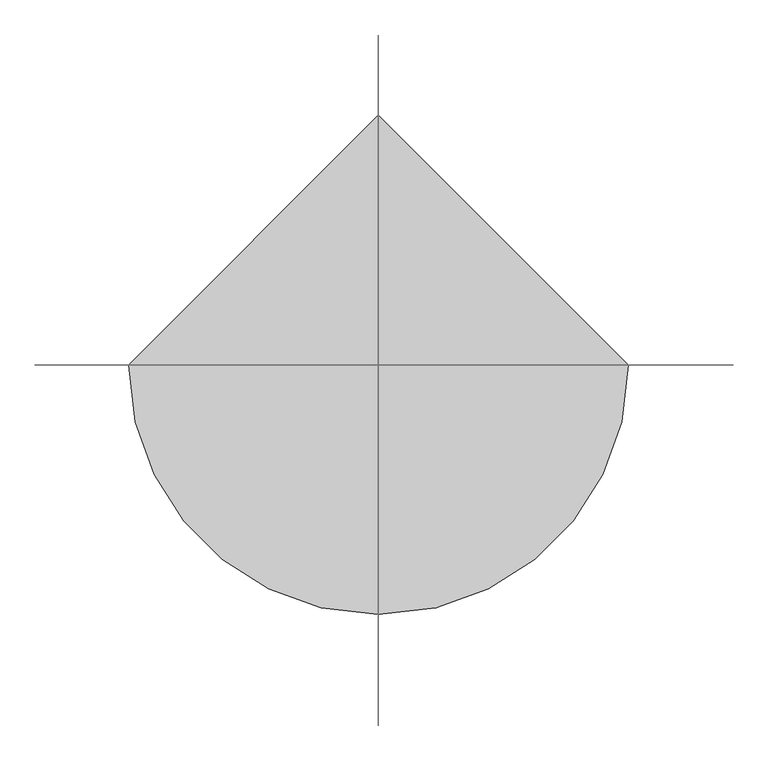
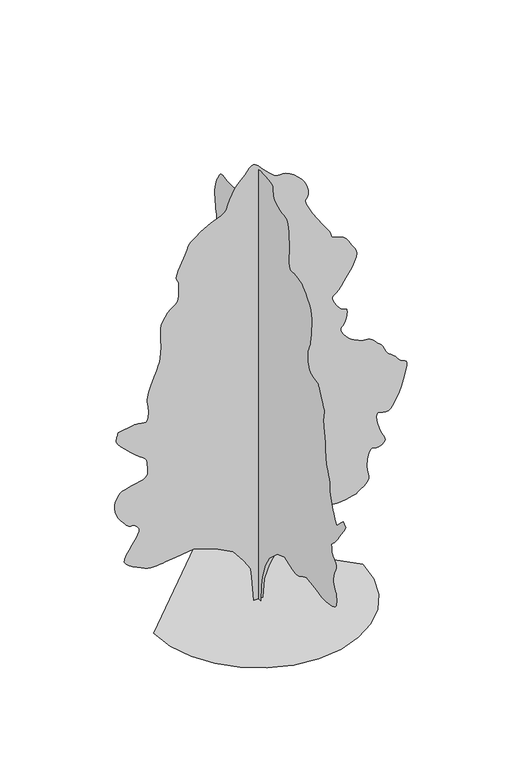
"""IFC4 building model written with IfcOpenShell, lengths in millimetres: geographic element geometry, RPC 木 - 落葉樹 : セイヨウハコヤナギ - 12.2 メートル."""

from ifc_helpers import new_model, si_unit, origin, place, context, project, spatial, triangles, source, transform, mapped, element, save


def geographic_element_e292760b(model_context):
    return source(origin(), model_context, "Body", "Tessellation", [
        triangles([(0.0009702, 113.8903775, 0.0), (0.0009702, -104.9033079, 0.0), (0.0009702, -123.1361794, 437.5878977), (0.0009702, -177.8345485, 729.312315), (0.0009702, -323.695976, 1130.4323805), (0.0009702, -506.0246724, 1440.3907139), (0.0009702, -870.6795582, 1768.5802746), (0.0009702, -1217.1031076, 1896.2099842), (0.0009702, -1399.4317314, 1823.2794067), (0.0009702, -1477.3592422, 1796.3301796), (0.0009702, -1554.013139, 1771.7701962), (0.0009702, -1628.1128311, 1751.9959671), (0.0009702, -1698.3871754, 1739.3994976), (0.0009702, -1763.5554359, 1736.3672699), (0.0009702, -1822.3466148, 1745.2987015), (0.0009702, -1873.4849178, 1768.5802746), (0.0009702, -1920.3683933, 1798.2415455), (0.0009702, -1967.2544849, 1825.0332241), (0.0009702, -2014.1379604, 1849.4331882), (0.0009702, -2061.0214359, 1871.9166996), (0.0009702, -2107.9050568, 1892.969339), (0.0009702, -2154.791003, 1913.0611359), (0.0009702, -2201.6746239, 1932.6776711), (0.0009702, -2584.5657875, 1877.9785389), (0.0009702, -2650.9541771, 1862.4566666), (0.0009702, -2717.1899597, 1847.5726913), (0.0009702, -2783.0952393, 1833.9646557), (0.0009702, -2848.5429886, 1822.2704567), (0.0009702, -2913.3300224, 1813.1255207), (0.0009702, -2977.329023, 1807.1729771), (0.0009702, -3040.387674, 1805.045636), (0.0009702, -3113.6893044, 1807.4372051), (0.0009702, -3202.6219574, 1815.2528618), (0.0009702, -3298.2393768, 1829.4456001), (0.0009702, -3391.6453033, 1850.9733559), (0.0009702, -3473.8681915, 1880.7947914), (0.0009702, -3536.0117821, 1919.8652264), (0.0009702, -3569.1298187, 1969.1428871), (0.0009702, -3581.5837097, 2022.7771133), (0.0009702, -3588.2684761, 2074.4973576), (0.0009702, -3590.1747551, 2124.6265652), (0.0009702, -3588.2684761, 2173.4773624), (0.0009702, -3583.4899887, 2221.3724041), (0.0009702, -3576.7802238, 2268.6270779), (0.0009702, -3569.1298187, 2315.5638931), (0.0009702, -3534.359848, 2355.0613369), (0.0009702, -3502.0042648, 2397.1080437), (0.0009702, -3474.4018799, 2444.2583633), (0.0009702, -3453.9923698, 2499.0617043), (0.0009702, -3443.1648331, 2564.0801193), (0.0009702, -3444.2577896, 2641.8294434), (0.0009702, -3459.736496, 2734.9307373), (0.0009702, -3486.8051926, 2827.040522), (0.0009702, -3517.6864471, 2902.5786438), (0.0009702, -3547.2968491, 2965.0274483), (0.0009702, -3570.5276985, 3017.919278), (0.0009702, -3582.270005, 3064.7620583), (0.0009702, -3577.4156502, 3109.0378441), (0.0009702, -3550.9059311, 3154.2795593), (0.0009702, -3512.094928, 3195.2003174), (0.0009702, -3474.8849899, 3227.1998177), (0.0009702, -3440.8774727, 3254.7513336), (0.0009702, -3411.622863, 3282.2775604), (0.0009702, -3388.7733856, 3314.2770607), (0.0009702, -3373.8792366, 3355.1981094), (0.0009702, -3368.5670609, 3409.5386879), (0.0009702, -3364.9071098, 3462.7866005), (0.0009702, -3357.1040977, 3500.758992), (0.0009702, -3349.9112228, 3528.1834808), (0.0009702, -3348.1575508, 3549.8638435), (0.0009702, -3356.6212784, 3570.6038567), (0.0009702, -3380.0553131, 3595.1564278), (0.0009702, -3423.2637222, 3628.3250427), (0.0009702, -3483.805957, 3682.2845398), (0.0009702, -3554.8963852, 3763.0330994), (0.0009702, -3634.7298843, 3866.097448), (0.0009702, -3721.578653, 3987.029892), (0.0009702, -3813.7140175, 4121.3568672), (0.0009702, -3909.3311462, 4264.6048096), (0.0009702, -4006.7278175, 4412.3263161), (0.0009702, -3897.3344948, 4521.744928), (0.0009702, -3751.468689, 4394.1024284), (0.0009702, -3605.6025925, 4230.012735), (0.0009702, -3582.0921089, 4261.5802849), (0.0009702, -3558.302282, 4295.0794029), (0.0009702, -3533.825869, 4332.3910789), (0.0009702, -3508.4346863, 4375.4468811), (0.0009702, -3481.7473618, 4426.1527977), (0.0009702, -3453.4586815, 4486.4412689), (0.0009702, -3423.2637222, 4558.1924126), (0.0009702, -3392.2298607, 4631.6207794), (0.0009702, -3362.4671425, 4698.9495186), (0.0009702, -3335.2458389, 4765.3631973), (0.0009702, -3311.8626732, 4835.8943573), (0.0009702, -3293.5626274, 4915.6772781), (0.0009702, -3281.6677139, 5009.820369), (0.0009702, -3277.3976257, 5123.4070404), (0.0009702, -3269.2135323, 5238.2901443), (0.0009702, -3247.6349075, 5336.8812195), (0.0009702, -3217.1347343, 5425.3060547), (0.0009702, -3182.1615784, 5509.5363785), (0.0009702, -3147.1628426, 5595.7241409), (0.0009702, -3116.6629601, 5689.8422333), (0.0009702, -3095.0843353, 5798.0408615), (0.0009702, -3081.5880661, 5895.9965103), (0.0009702, -3071.9043549, 5963.3505386), (0.0009702, -3065.4230644, 6011.8708328), (0.0009702, -3061.4834793, 6053.4014374), (0.0009702, -3059.4754623, 6099.6852402), (0.0009702, -3058.7130089, 6162.5657043), (0.0009702, -3058.6112709, 6253.8368774), (0.0009702, -3054.5702385, 6347.2939636), (0.0009702, -3044.1493629, 6416.5036926), (0.0009702, -3029.9159294, 6472.9537354), (0.0009702, -3014.3863541, 6528.1335068), (0.0009702, -3000.1532112, 6593.5300964), (0.0009702, -2989.7323357, 6680.582341), (0.0009702, -2985.6910126, 6800.8284897), (0.0009702, -2991.2572426, 6913.2716263), (0.0009702, -3003.5335281, 6981.3628189), (0.0009702, -3015.8351028, 7023.299794), (0.0009702, -3021.4013329, 7057.2564423), (0.0009702, -3013.5986115, 7101.4304901), (0.0009702, -2985.6910126, 7173.9952469), (0.0009702, -2930.9943512, 7293.1228592), (0.0009702, -2868.6219955, 7422.976561), (0.0009702, -2820.6353897, 7519.3561432), (0.0009702, -2784.5945663, 7587.8287079), (0.0009702, -2758.1107178, 7633.959613), (0.0009702, -2738.8194534, 7663.3671204), (0.0009702, -2724.3063858, 7681.5904266), (0.0009702, -2712.1827072, 7694.2483749), (0.0009702, -2638.2965195, 7706.295314), (0.0009702, -2566.4945068, 7720.4525894), (0.0009702, -2498.8204399, 7738.7270554), (0.0009702, -2437.3730278, 7763.2290482), (0.0009702, -2384.2142086, 7796.0415802), (0.0009702, -2341.425396, 7839.199411), (0.0009702, -2311.0702721, 7894.8105515), (0.0009702, -2290.8183105, 7956.2428482), (0.0009702, -2276.3080044, 8015.7938644), (0.0009702, -2266.578511, 8073.7182358), (0.0009702, -2260.6793072, 8130.3973343), (0.0009702, -2257.6495502, 8186.1107941), (0.0009702, -2256.5313046, 8241.1632477), (0.0009702, -2256.3736107, 8295.9104874), (0.0009702, -2287.4709858, 8351.2169952), (0.0009702, -2317.6099892, 8410.0058487), (0.0009702, -2345.8351559, 8475.8093903), (0.0009702, -2371.1907303, 8552.1355453), (0.0009702, -2392.7211021, 8642.5172379), (0.0009702, -2409.4655743, 8750.4106522), (0.0009702, -2420.4685364, 8879.374292), (0.0009702, -2431.6848576, 9010.8290588), (0.0009702, -2445.4530579, 9127.2882294), (0.0009702, -2455.3934395, 9233.8857925), (0.0009702, -2455.1265953, 9335.6789978), (0.0009702, -2438.2754436, 9437.7779984), (0.0009702, -2398.4602867, 9545.3156204), (0.0009702, -2329.3041882, 9663.375856), (0.0009702, -2249.3561611, 9774.6498779), (0.0009702, -2178.6572788, 9861.3457489), (0.0009702, -2113.0620094, 9927.9370331), (0.0009702, -2048.4224957, 9978.9234558), (0.0009702, -1980.5956764, 10018.7256775), (0.0009702, -1905.4310783, 10051.8434235), (0.0009702, -1818.7857857, 10082.7252594), (0.0009702, -1726.6658272, 10101.4566742), (0.0009702, -1639.9671947, 10102.9310028), (0.0009702, -1561.8796646, 10098.9917084), (0.0009702, -1495.593013, 10101.4566742), (0.0009702, -1444.2971615, 10122.0693695), (0.0009702, -1411.1794155, 10172.6744202), (0.0009702, -1399.4317314, 10265.0641296), (0.0009702, -1401.3457134, 10369.4751984), (0.0009702, -1405.8114292, 10455.052533), (0.0009702, -1410.9150421, 10532.0141144), (0.0009702, -1414.7402447, 10610.5767609), (0.0009702, -1415.3781418, 10700.9584534), (0.0009702, -1410.9150421, 10813.3260132), (0.0009702, -1399.4317314, 10957.9206757), (0.0009702, -1383.5921459, 11104.7268311), (0.0009702, -1366.4740047, 11219.3303009), (0.0009702, -1346.8067459, 11305.2390106), (0.0009702, -1323.3115231, 11365.9341431), (0.0009702, -1294.7128326, 11404.9480408), (0.0009702, -1259.7344444, 11425.7897919), (0.0009702, -1217.1031076, 11431.9661591), (0.0009702, -1156.2404709, 11437.4821014), (0.0009702, -1074.0049381, 11453.8752869), (0.0009702, -980.2913269, 11480.7666687), (0.0009702, -884.9789761, 11517.8748688), (0.0009702, -797.9626305, 11564.8440948), (0.0009702, -729.1241724, 11621.4220367), (0.0009702, -688.3534052, 11687.2249969), (0.0009702, -673.3092653, 11757.0707336), (0.0009702, -668.4724966, 11824.0433899), (0.0009702, -663.953441, 11885.2722107), (0.0009702, -649.8675276, 11937.9096954), (0.0009702, -616.3252436, 11979.0595093), (0.0009702, -553.4419453, 12005.8485718), (0.0009702, -451.3255766, 12015.4049652), (0.0009702, -328.0015635, 12019.0907867), (0.0009702, -210.419678, 12026.8937988), (0.0009702, -102.0858745, 12034.0608032), (0.0009702, -6.5099094, 12035.8141846), (0.0009702, 72.8000803, 12027.3763275), (0.0009702, 132.3357269, 12003.9417114), (0.0009702, 168.5887284, 11960.7083038), (0.0009702, 190.3829832, 11911.6031616), (0.0009702, 211.2205557, 11869.1836578), (0.0009702, 234.6091899, 11826.7629913), (0.0009702, 264.0584098, 11777.6322693), (0.0009702, 303.0754686, 11715.1325958), (0.0009702, 355.1693819, 11632.5283356), (0.0009702, 423.847639, 11523.1361755), (0.0009702, 499.9145439, 11406.6002655), (0.0009702, 572.4739231, 11305.3913269), (0.0009702, 642.4814959, 11216.9420746), (0.0009702, 710.8954159, 11138.6840607), (0.0009702, 778.6688227, 11068.1023224), (0.0009702, 846.7624861, 11002.602832), (0.0009702, 916.132089, 10939.6717896), (0.0009702, 984.3859171, 10887.6947296), (0.0009702, 1049.1322557, 10854.1956116), (0.0009702, 1111.3241718, 10835.3874573), (0.0009702, 1171.9250513, 10827.4065491), (0.0009702, 1231.8854176, 10826.440329), (0.0009702, 1292.1634243, 10828.6774017), (0.0009702, 1353.7199867, 10830.2784668), (0.0009702, 1420.0599781, 10835.869986), (0.0009702, 1491.5035824, 10848.1459808), (0.0009702, 1564.2205101, 10860.4231384), (0.0009702, 1634.3881748, 10865.9890778), (0.0009702, 1698.1762871, 10858.1860657), (0.0009702, 1751.7570282, 10830.2784668), (0.0009702, 1791.3078117, 10775.5818054), (0.0009702, 1825.3814587, 10707.9731415), (0.0009702, 1862.9624496, 10643.2119781), (0.0009702, 1900.8637699, 10577.5101746), (0.0009702, 1935.8928818, 10507.0295929), (0.0009702, 1964.8627705, 10427.9332581), (0.0009702, 1984.5861305, 10336.4086121), (0.0009702, 1991.8679535, 10228.5907745), (0.0009702, 1989.7406124, 10117.6475464), (0.0009702, 1983.7879234, 10017.5559814), (0.0009702, 1974.6456036, 9925.75112), (0.0009702, 1962.9514046, 9839.6912567), (0.0009702, 1949.3433689, 9756.8323608), (0.0009702, 1934.4593937, 9674.610054), (0.0009702, 1918.9375214, 9590.455307), (0.0009702, 1915.5875805, 9511.6130264), (0.0009702, 1932.3320526, 9444.2589981), (0.0009702, 1962.471056, 9384.2504517), (0.0009702, 1999.3099411, 9327.4190369), (0.0009702, 2036.1488262, 9269.6469818), (0.0009702, 2066.2878296, 9206.7659363), (0.0009702, 2083.0323017, 9134.6337112), (0.0009702, 2082.5544239, 9064.6106598), (0.0009702, 2068.0415016, 9007.7030869), (0.0009702, 2043.3239697, 8959.0554749), (0.0009702, 2012.2265945, 8913.9157883), (0.0009702, 1978.5801018, 8867.505249), (0.0009702, 1946.2069324, 8815.045079), (0.0009702, 1918.9375214, 8751.7320831), (0.0009702, 1903.0953197, 8679.3963821), (0.0009702, 1901.6083466, 8603.858551), (0.0009702, 1913.195866, 8526.4138596), (0.0009702, 1936.584264, 8448.3337418), (0.0009702, 1970.4976009, 8370.8640518), (0.0009702, 2013.6626987, 8295.3256393), (0.0009702, 2064.7983856, 8222.9899384), (0.0009702, 2117.5836811, 8163.4133423), (0.0009702, 2167.8170975, 8119.112558), (0.0009702, 2217.4124714, 8080.9114014), (0.0009702, 2268.2839302, 8039.4819534), (0.0009702, 2322.3450199, 7985.6497742), (0.0009702, 2381.5073971, 7910.1113617), (0.0009702, 2447.6872238, 7803.6411163), (0.0009702, 2517.1100212, 7689.1899628), (0.0009702, 2585.5825859, 7593.5731247), (0.0009702, 2654.3597832, 7513.2309357), (0.0009702, 2724.7386269, 7444.7333725), (0.0009702, 2797.9893883, 7384.4957703), (0.0009702, 2875.3829201, 7329.0619446), (0.0009702, 2958.2156548, 7274.8739731), (0.0009702, 3041.988739, 7232.046936), (0.0009702, 3121.6190529, 7206.7316208), (0.0009702, 3197.4115196, 7189.7280075), (0.0009702, 3269.6963516, 7171.7587555), (0.0009702, 3338.8043427, 7143.5971024), (0.0009702, 3405.0398346, 7095.9662888), (0.0009702, 3468.7339119, 7019.6145538), (0.0009702, 3527.5736343, 6926.1324692), (0.0009702, 3577.7967316, 6834.2258698), (0.0009702, 3617.5230858, 6745.496402), (0.0009702, 3644.7696785, 6661.5707108), (0.0009702, 3657.7066795, 6583.9992828), (0.0009702, 3654.3516518, 6514.4337616), (0.0009702, 3632.823896, 6454.3996353), (0.0009702, 3592.3603775, 6396.7293182), (0.0009702, 3536.9268425, 6334.585437), (0.0009702, 3471.6061203, 6270.2306442), (0.0009702, 3401.4816216, 6205.8502716), (0.0009702, 3331.6876259, 6143.7069717), (0.0009702, 3267.3072533, 6086.0366547), (0.0009702, 3213.4747833, 6035.0508133), (0.0009702, 3163.8615326, 5989.0210648), (0.0009702, 3111.4016533, 5943.6273239), (0.0009702, 3059.8821236, 5897.267363), (0.0009702, 3013.1663704, 5848.3656967), (0.0009702, 2975.0669518, 5795.3212601), (0.0009702, 2949.3705551, 5736.5324066), (0.0009702, 2939.966478, 5670.3986526), (0.0009702, 2936.1033417, 5601.0871857), (0.0009702, 2926.8007118, 5533.3517853), (0.0009702, 2915.5665138, 5466.6081848), (0.0009702, 2905.9589607, 5400.1436371), (0.0009702, 2901.4348183, 5333.3738754), (0.0009702, 2905.5270103, 5265.6640549), (0.0009702, 2921.742881, 5196.3531693), (0.0009702, 2946.7782715, 5129.7357239), (0.0009702, 2974.6855797, 5069.8289154), (0.0009702, 3004.9822769, 5015.5136261), (0.0009702, 3037.1852531, 4965.6463211), (0.0009702, 3070.8366875, 4919.1340439), (0.0009702, 3105.4543419, 4874.8579674), (0.0009702, 3140.5292358, 4831.7007179), (0.0009702, 3183.2289551, 4838.4869316), (0.0009702, 3224.1497131, 4839.2493851), (0.0009702, 3261.5631271, 4827.8625801), (0.0009702, 3293.7405235, 4798.3030472), (0.0009702, 3318.877652, 4744.5214462), (0.0009702, 3335.2458389, 4660.4178589), (0.0009702, 3341.091703, 4539.9685249), (0.0009702, 3341.091703, 3938.2808327), (0.0009702, 3347.8017586, 3760.1103127), (0.0009702, 3363.4330719, 3613.5070518), (0.0009702, 3381.2752968, 3494.3285706), (0.0009702, 3394.6701187, 3398.431517), (0.0009702, 3396.9066101, 3321.6734116), (0.0009702, 3381.2752968, 3259.8856133), (0.0009702, 3341.091703, 3208.9762207), (0.0009702, 3283.7263092, 3180.3314575), (0.0009702, 3223.8195007, 3176.2395561), (0.0009702, 3165.5137573, 3178.8321304), (0.0009702, 3112.95214, 3170.2666649), (0.0009702, 3070.2521301, 3132.7009346), (0.0009702, 3041.6076576, 3048.2159752), (0.0009702, 3031.1359131, 2899.0204308), (0.0009702, 3038.0494446, 2734.6002342), (0.0009702, 3055.1547958, 2610.6941345), (0.0009702, 3077.0639236, 2518.6782394), (0.0009702, 3098.3376251, 2449.9466789), (0.0009702, 3113.5366974, 2395.8855892), (0.0009702, 3117.2475174, 2347.8837227), (0.0009702, 3104.0561714, 2297.3325932), (0.0009702, 3091.0938812, 2255.6569393), (0.0009702, 3091.8307549, 2234.0756985), (0.0009702, 3095.4654167, 2223.657439), (0.0009702, 3091.0938812, 2215.4707294), (0.0009702, 3067.9139008, 2200.5867542), (0.0009702, 3015.0726494, 2170.0740818), (0.0009702, 2921.742881, 2115.0038967), (0.0009702, 2824.1938934, 2054.1920563), (0.0009702, 2755.3655365, 2010.2848526), (0.0009702, 2699.2709953, 1980.0923641), (0.0009702, 2639.9996132, 1960.4249599), (0.0009702, 2561.6145721, 1948.0928638), (0.0009702, 2448.1142326, 1939.9061543), (0.0009702, 2283.5922981, 1932.6776711), (0.0009702, 2107.2721012, 1934.962706), (0.0009702, 1964.7585617, 1953.194006), (0.0009702, 1849.6721272, 1980.9972507), (0.0009702, 1755.6381866, 2011.9851849), (0.0009702, 1676.2747169, 2039.7859589), (0.0009702, 1605.2047817, 2058.0197296), (0.0009702, 1536.0486832, 2060.3047646), (0.0009702, 1461.4686424, 2050.3642376), (0.0009702, 1379.2357258, 2036.5986534), (0.0009702, 1290.6232567, 2019.6406769), (0.0009702, 1196.9070293, 2000.1334373), (0.0009702, 1099.3656721, 1978.709745), (0.0009702, 999.2698923, 1956.0127293), (0.0009702, 897.9007891, 1932.6776711), (0.0009702, 533.2433599, 1640.9507103), (0.0009702, 314.4519545, 1166.90014), (0.0009702, 168.5887284, 601.6827144), (120.2564769, 0.0005338, 0.0085401), (-116.7693169, 0.0005338, 0.0085401), (-171.467677, 0.0004852, 656.3894405), (-207.9336742, 0.0004852, 911.6486418), (-390.2621163, 0.000461, 1203.3730591), (-663.7526539, 0.0004367, 1549.7965359), (-1137.8057676, 0.0004124, 1805.0556644), (-1721.2571457, 0.0004124, 1987.3818901), (-2195.307716, 0.0004124, 1932.6853741), (-2468.8007607, 0.0004124, 1896.220158), (-2535.4583199, 0.0004124, 1886.7041691), (-2609.1436478, 0.0004124, 1875.9122406), (-2687.9097702, 0.0004124, 1867.0367649), (-2769.8786041, 0.0004124, 1863.262286), (-2853.118, 0.0004124, 1867.7814869), (-2935.7219696, 0.0004124, 1883.781237), (-3015.7842339, 0.0004124, 1914.451458), (-3106.3182426, 0.0004124, 1956.8718338), (-3213.0937019, 0.0004124, 2005.9868591), (-3323.4017944, 0.0004124, 2061.8043823), (-3424.4581261, 0.0004124, 2124.316555), (-3503.5038826, 0.0003882, 2193.5259933), (-3547.7796684, 0.0003882, 2269.4326973), (-3544.5263786, 0.0003882, 2352.039283), (-3497.4801224, 0.0003882, 2448.838607), (-3427.1777275, 0.0003882, 2561.589283), (-3345.9972176, 0.0003639, 2681.6572449), (-3266.4177727, 0.0003639, 2800.4802246), (-3200.8682854, 0.0003639, 2909.3904373), (-3161.8029373, 0.0003397, 2999.797419), (-3161.6503304, 0.0003397, 3063.1101242), (-3185.0843651, 0.0003397, 3105.2255768), (-3208.5186905, 0.0003397, 3138.699115), (-3231.9783051, 0.0003397, 3165.0306473), (-3255.4123398, 0.0003397, 3185.5927643), (-3278.8463745, 0.0003397, 3201.8595039), (-3302.3059891, 0.0003397, 3215.2540352), (-3325.7400238, 0.0003397, 3227.2253975), (-3349.3522453, 0.0003397, 3223.6924736), (-3373.9045258, 0.0003397, 3222.5995171), (-3400.3633759, 0.0003397, 3226.2594681), (-3429.7194328, 0.0003397, 3237.112294), (-3462.8883385, 0.0003397, 3257.521804), (-3500.8351501, 0.0003397, 3289.8770966), (-3544.5263786, 0.0003397, 3336.6184296), (-3595.9950394, 0.0003397, 3397.7455124), (-3652.5471107, 0.0003154, 3470.6657707), (-3708.1585419, 0.0003154, 3553.8034286), (-3756.729705, 0.0003154, 3645.5574211), (-3792.2368401, 0.0003154, 3744.3263924), (-3808.6306068, 0.0002911, 3848.5092773), (-3799.7855072, 0.0002911, 3956.5300095), (-3773.9115051, 0.0002911, 4054.2313133), (-3742.2677971, 0.0002911, 4130.8879715), (-3703.6343994, 0.0002911, 4189.9817482), (-3656.6898811, 0.0002669, 4235.0708565), (-3600.1886787, 0.0002669, 4269.6120621), (-3532.8346504, 0.0002669, 4297.163578), (-3453.3825233, 0.0002669, 4321.1821701), (-3359.0103767, 0.0002669, 4341.1597298), (-3254.4719902, 0.0002669, 4358.2906609), (-3149.5775208, 0.0002669, 4378.5984329), (-3054.2650246, 0.0002669, 4408.1579659), (-2978.4219795, 0.0002669, 4453.018309), (-2931.9094116, 0.0002669, 4519.2540916), (-2924.6147987, 0.0002669, 4612.9143631), (-2935.5184937, 0.0002426, 4710.7174049), (-2940.34785, 0.0002426, 4788.1112274), (-2944.2365662, 0.0002426, 4849.2380196), (-2952.2680527, 0.0002426, 4898.2411331), (-2969.5260109, 0.0002426, 4939.289209), (-3001.1697189, 0.0002426, 4976.499147), (-3052.2572983, 0.0002426, 5014.0392975), (-3137.5552895, 0.0002184, 5075.3698563), (-3257.0134048, 0.0002184, 5172.1052307), (-3393.3483971, 0.0002184, 5290.5468384), (-3529.3781754, 0.0002184, 5416.9437744), (-3647.8703613, 0.0001941, 5537.6218735), (-3731.5928673, 0.0001941, 5638.8308121), (-3763.3380226, 0.0001941, 5706.8714264), (-3761.7369576, 0.0001941, 5751.0960526), (-3757.2636841, 0.0001941, 5790.5430634), (-3750.4010216, 0.0001941, 5825.9990387), (-3741.6323708, 0.0001698, 5858.2528839), (-3731.4402603, 0.0001698, 5888.1429199), (-3720.2825111, 0.0001698, 5916.4057297), (-3708.6416519, 0.0001698, 5943.906958), (-3271.0436531, 0.0001698, 6016.8269257), (-3176.2139763, 0.0001698, 6018.4285721), (-3095.0843353, 0.0001698, 6002.7969681), (-3028.0096504, 0.0001698, 5986.1997253), (-2975.270137, 0.0001698, 5984.929454), (-2937.2215874, 0.0001698, 6015.2258606), (-2914.1433449, 0.0001698, 6093.3821365), (-2906.3912018, 0.0001698, 6235.6135712), (-2912.8724922, 0.0001456, 6381.32677), (-2927.0041878, 0.0001456, 6474.7326965), (-2940.8306694, 0.0001456, 6539.4182831), (-2946.3716103, 0.0001456, 6598.9948792), (-2935.6202316, 0.0001213, 6677.0999954), (-2900.6470757, 0.0001213, 6797.269986), (-2833.4453636, 0.0001213, 6983.1673599), (-2756.1535698, 9.7e-05, 7180.2733521), (-2695.1535141, 9.7e-05, 7329.8496872), (-2648.7935532, 9.7e-05, 7449.1301971), (-2615.5232002, 7.28e-05, 7555.3463882), (-2593.7158104, 7.28e-05, 7665.7053497), (-2581.8208969, 7.28e-05, 7797.4141708), (-2578.186235, 4.85e-05, 7967.7311005), (-2581.6938698, 4.85e-05, 8141.3013199), (-2588.4036346, 4.85e-05, 8277.8644958), (-2592.5466957, 2.43e-05, 8387.3083969), (-2588.4036346, 2.43e-05, 8479.5457901), (-2570.2309067, 2.43e-05, 8564.4371201), (-2532.2710144, 2.43e-05, 8651.8701553), (-2468.8007607, 0.0, 8751.757663), (-2395.1256065, 0.0, 8844.6043213), (-2330.3792679, 0.0, 8909.7218582), (-2274.5643608, 0.0, 8955.0650208), (-2227.6808853, 0.0, 8988.6152985), (-2189.7262253, 0.0, 9018.3274384), (-2160.7029968, 0.0, 9052.1823486), (-2140.6085838, 0.0, 9098.1609375), (-2127.1072277, -2.43e-05, 9141.3437668), (-2117.4336903, -2.43e-05, 9168.8699936), (-2110.9473129, -2.43e-05, 9191.9482361), (-2107.0154308, -2.43e-05, 9221.7109543), (-2104.9947693, -2.43e-05, 9269.3417679), (-2104.2500473, -2.43e-05, 9345.9981354), (-2104.1458385, -2.43e-05, 9462.838678), (-2114.4574184, -4.85e-05, 9573.8330658), (-2137.5281033, -4.85e-05, 9640.805722), (-2161.5543983, -4.85e-05, 9686.7337326), (-2174.7354252, -4.85e-05, 9734.5680222), (-2165.2753922, -4.85e-05, 9807.2850952), (-2121.3657177, -7.28e-05, 9927.8358765), (-2031.2129356, -7.28e-05, 10119.1974518), (-1940.7398243, -7.28e-05, 10312.5926239), (-1890.135355, -9.7e-05, 10438.3535522), (-1858.9847855, -9.7e-05, 10518.2126312), (-1826.8784603, -9.7e-05, 10573.7987732), (-1773.4019279, -9.7e-05, 10626.8687897), (-1678.1453876, -9.7e-05, 10699.0527557), (-1520.6945332, -0.0001213, 10812.0551605), (-1342.5671791, -0.0001213, 10924.4727173), (-1196.3326458, -0.0001213, 10992.5894897), (-1078.165658, -0.0001213, 11034.5264648), (-984.2359989, -0.0001213, 11068.4836945), (-910.7209368, -0.0001213, 11112.6577423), (-853.7901821, -0.0001456, 11185.2219177), (-809.6161343, -0.0001456, 11304.34953), (-760.4450804, -0.0001456, 11447.9791351), (-695.3276888, -0.0001698, 11580.450119), (-620.643512, -0.0001698, 11699.5021545), (-542.7695226, -0.0001698, 11802.9470032), (-468.082766, -0.0001698, 11888.5255005), (-402.9678815, -0.0001698, 11954.0238281), (-353.7969003, -0.0001941, 11997.1816589), (-315.471151, -0.0001941, 12037.7466248), (-277.1428946, -0.0001941, 12089.4690491), (-236.5850686, -0.0001941, 12141.1914734), (-191.5607819, -0.0001941, 12181.7564392), (-139.8392296, -0.0001941, 12199.9809082), (-79.1872813, -0.0001941, 12184.7306763), (-7.3724481, -0.0001941, 12124.8238678), (68.5354242, -0.0001941, 12043.2102448), (139.978002, -0.0001941, 11969.908905), (206.9556453, -0.0001698, 11904.2582611), (269.4670731, -0.0001698, 11845.6467224), (327.5160916, -0.0001698, 11793.3906097), (381.0969054, -0.0001698, 11746.8783325), (430.2145105, -0.0001698, 11705.4750458), (477.6292399, -0.0001698, 11680.1091522), (528.236289, -0.0001698, 11674.5176331), (585.2203471, -0.0001698, 11677.2372345), (651.7712631, -0.0001698, 11676.7535431), (731.0813204, -0.0001698, 11661.6056305), (826.3377153, -0.0001698, 11620.3035004), (940.7328403, -0.0001456, 11541.3594818), (1053.7962152, -0.0001456, 11441.8539276), (1144.2183849, -0.0001456, 11345.8551361), (1213.9057011, -0.0001456, 11252.3980499), (1264.7770145, -0.0001456, 11160.5420288), (1298.7438366, -0.0001213, 11069.3220154), (1317.7198586, -0.0001213, 10977.7962067), (1323.6216785, -0.0001213, 10884.9751282), (1311.5004707, -0.0001213, 10814.3933899), (1284.7112629, -0.0001213, 10775.7085419), (1257.5994003, -0.0001213, 10747.1916779), (1244.5225822, -9.7e-05, 10707.2371399), (1259.8335663, -9.7e-05, 10634.0881165), (1317.8800232, -9.7e-05, 10506.0889526), (1433.0173267, -7.28e-05, 10301.536322), (1569.3648182, -7.28e-05, 10081.0474548), (1682.1104073, -4.85e-05, 9912.86586), (1772.2123203, -4.85e-05, 9786.7735565), (1840.6236969, -4.85e-05, 9692.579306), (1888.3053795, -4.85e-05, 9620.0657089), (1916.212833, -4.85e-05, 9559.0403641), (1925.3042839, -2.43e-05, 9499.2858719), (1944.8650085, -2.43e-05, 9450.4859436), (1996.9589218, -2.43e-05, 9421.4603897), (2071.6965111, -2.43e-05, 9400.7459564), (2159.1932053, -2.43e-05, 9376.8288116), (2249.5594917, -2.43e-05, 9338.2207031), (2332.9107994, -2.43e-05, 9273.4845383), (2399.3574703, -2.43e-05, 9171.106485), (2456.2346672, 0.0, 9061.1794739), (2512.7942963, 0.0, 8974.8393951), (2562.0212334, 0.0, 8902.2240601), (2596.892942, 0.0, 8833.4468628), (2610.3892113, 0.0, 8758.594455), (2595.4950623, 2.43e-05, 8667.8063919), (2545.2208054, 2.43e-05, 8551.1949051), (2482.9731514, 2.43e-05, 8437.658812), (2433.4843117, 2.43e-05, 8355.0295532), (2391.6486385, 2.43e-05, 8291.8944534), (2352.3646992, 4.85e-05, 8236.7152634), (2310.5314968, 4.85e-05, 8178.0281479), (2261.0426571, 4.85e-05, 8104.3454361), (2198.7948578, 4.85e-05, 8004.2038742), (2128.4161594, 4.85e-05, 7909.2218811), (2062.1829929, 7.28e-05, 7849.3150726), (2006.4749107, 7.28e-05, 7810.4529099), (1967.6687038, 7.28e-05, 7778.6060165), (1952.1468315, 7.28e-05, 7739.7438538), (1966.2887009, 7.28e-05, 7679.8370453), (2016.4686321, 7.28e-05, 7584.8550522), (2082.0105618, 7.28e-05, 7483.0612656), (2138.9412437, 9.7e-05, 7408.9971817), (2188.6943115, 9.7e-05, 7358.0880798), (2232.7108109, 9.7e-05, 7325.6563385), (2272.4166721, 9.7e-05, 7307.1022385), (2309.2555573, 9.7e-05, 7297.7993179), (2344.6583382, 9.7e-05, 7293.1228592), (2348.379332, 9.7e-05, 7265.4187363), (2350.9845509, 9.7e-05, 7235.6560181), (2351.3556038, 9.7e-05, 7201.7499481), (2348.379332, 9.7e-05, 7161.617514), (2340.9373444, 9.7e-05, 7113.1983765), (2327.913866, 0.0001213, 7054.4101044), (2308.1931221, 0.0001213, 6983.1673599), (2279.3274422, 0.0001213, 6918.9648834), (2244.722723, 0.0001213, 6875.7820541), (2212.0318405, 0.0001213, 6843.4776306), (2188.9078159, 0.0001213, 6811.7830536), (2183.0086121, 0.0001213, 6770.5315018), (2201.984634, 0.0001213, 6709.5061569), (2253.4939899, 0.0001456, 6618.5146179), (2323.6616547, 0.0001456, 6523.7872604), (2392.871093, 0.0001456, 6454.5775314), (2460.1666946, 0.0001456, 6405.1421768), (2524.592704, 0.0001456, 6369.7367798), (2585.2012138, 0.0001456, 6342.6175049), (2641.0161209, 0.0001456, 6318.0649338), (2691.0869019, 0.0001456, 6290.3096512), (2740.0394371, 0.0001456, 6267.8924149), (2792.4993164, 0.0001456, 6258.2087036), (2847.5261902, 0.0001698, 6253.9641953), (2904.1291306, 0.0001698, 6247.7878281), (2961.3927864, 0.0001698, 6232.3852798), (3018.3259392, 0.0001698, 6200.3860703), (3073.9629501, 0.0001698, 6144.4691345), (3123.5000427, 0.0001698, 6088.0696701), (3164.4460899, 0.0001698, 6052.7154327), (3199.3177986, 0.0001698, 6028.2134399), (3230.6818726, 0.0001698, 6004.3474548), (3261.0803078, 0.0001698, 5970.8989151), (3293.079808, 0.0001698, 5917.7021622), (3329.2220787, 0.0001941, 5834.5136353), (3369.5329903, 0.0001941, 5750.0798355), (3412.6902397, 0.0001941, 5692.7903091), (3459.3554146, 0.0001941, 5651.7428146), (3510.1630692, 0.0001941, 5616.1339417), (3565.774791, 0.0001941, 5575.0858658), (3626.8001358, 0.0001941, 5517.7969208), (3693.87453, 0.0002184, 5433.3881195), (3762.397673, 0.0002184, 5358.4345551), (3824.5412636, 0.0002184, 5322.6989456), (3876.1625313, 0.0002184, 5305.161644), (3913.0928352, 0.0002184, 5284.7518433), (3931.240274, 0.0002184, 5240.4254791), (3926.3859192, 0.0002184, 5151.1111633), (3894.4369972, 0.0002426, 4995.7904114), (3842.409359, 0.0002426, 4804.5811523), (3781.7398064, 0.0002669, 4624.8601456), (3715.0464935, 0.0002669, 4461.4058784), (3644.8205475, 0.0002669, 4318.9965477), (3573.6539612, 0.0002911, 4202.4356392), (3504.0631508, 0.0002911, 4116.4766418), (3438.6154015, 0.0002911, 4065.9230415), (3370.8038429, 0.0002911, 4054.7144234), (3297.8580048, 0.0002911, 4069.9643646), (3228.1148781, 0.0002911, 4091.2889351), (3169.8600037, 0.0002911, 4098.2530449), (3131.379213, 0.0002911, 4070.447184), (3120.9583374, 0.0002911, 3987.4618423), (3146.9087883, 0.0002911, 3828.8875099), (3198.9364265, 0.0003154, 3650.9204659), (3255.1327057, 0.0003154, 3516.9748627), (3306.2199944, 0.0003154, 3417.4687271), (3342.947113, 0.0003397, 3342.8200859), (3356.0620102, 0.0003397, 3283.4975441), (3336.3643753, 0.0003397, 3229.9194191), (3274.525708, 0.0003397, 3172.5031563), (3194.0056229, 0.0003397, 3136.3100166), (3123.6779388, 0.0003397, 3137.4282623), (3062.601725, 0.0003397, 3152.9069687), (3009.8113426, 0.0003397, 3159.7696312), (2964.3664421, 0.0003397, 3135.039164), (2925.3010941, 0.0003397, 3055.7902222), (2891.6496597, 0.0003639, 2899.0204308), (2877.9754944, 0.0003639, 2720.9007797), (2889.5146156, 0.0003882, 2585.811351), (2911.2458473, 0.0003882, 2483.2830162), (2928.2241714, 0.0003882, 2402.7505772), (2925.402832, 0.0003882, 2333.7011581), (2887.8115219, 0.0003882, 2265.6074947), (2800.4802246, 0.0003882, 2187.9445026), (2703.3631874, 0.0004124, 2116.5008984), (2637.5087769, 0.0004124, 2069.6174229), (2589.4965912, 0.0004124, 2040.5941944), (2545.9579697, 0.0004124, 2022.7339474), (2493.4954742, 0.0004124, 2009.3368), (2418.7045452, 0.0004124, 1993.7081028), (2308.1931221, 0.0004124, 1969.1505901), (2183.5398296, 0.0004124, 1948.1539066), (2072.2835392, 0.0004124, 1944.0592438), (1969.9562096, 0.0004124, 1951.4503624), (1872.0945957, 0.0004124, 1964.8983788), (1774.2329819, 0.0004124, 1978.9842922), (1671.9056522, 0.0004124, 1988.2867767), (1560.6495071, 0.0004124, 1987.3818901), (1455.6634735, 0.0004124, 1977.4415085), (1372.6858349, 0.0004124, 1963.675779), (1308.0463211, 0.0004124, 1946.7178024), (1258.0797489, 0.0004124, 1927.2105629), (1219.1160662, 0.0004124, 1905.7868706), (1187.4876188, 0.0004124, 1883.0898548), (1159.5268255, 0.0004124, 1859.7547966), (1159.2065689, 0.0004367, 1762.4244003), (1156.9749464, 0.0004367, 1667.1653893), (1150.9131071, 0.0004367, 1576.0569969), (1139.1146994, 0.0004367, 1491.1655216), (1119.6582561, 0.0004367, 1414.5648193), (1090.6350277, 0.000461, 1348.3316528), (1050.1285612, 0.000461, 1294.5374073), (1004.8386658, 0.000461, 1252.4372154), (962.4209061, 0.000461, 1218.9483438), (922.3922447, 0.000461, 1192.6370138), (884.2800362, 0.000461, 1172.0648684), (847.601243, 0.000461, 1155.7982014), (811.8807489, 0.000461, 1142.401054), (776.63806, 0.000461, 1130.4425543), (466.6797629, 0.000461, 1130.4425543), (284.3510483, 0.0004852, 856.9495096), (156.7227194, 0.0005095, 510.5259602), (-2767.8705872, 0.0, 0.0100928), (-2694.6959839, -634.216012, 0.0100928), (-2486.310157, -1216.6404905, 0.0100928), (-2159.3761883, -1730.5901516, 0.0100928), (-1730.5901516, -2159.3761883, 0.0100928), (-1216.6404905, -2486.310157, 0.0100928), (-634.216012, -2694.6959839, 0.0100928), (0.000121, -2767.8705872, 0.0100928), (634.216012, -2694.6959839, 0.0100928), (1216.6404905, -2486.310157, 0.0100928), (1730.5901516, -2159.3761883, 0.0100928), (2159.3761883, -1730.5901516, 0.0100928), (2486.310157, -1216.6404905, 0.0100928), (2694.6959839, -634.216012, 0.0100928), (2767.8705872, 0.0002426, 0.0100928), (-0.000363, 2767.8705872, 0.0100928)], [[1, 2, 3], [388, 1, 3], [388, 3, 4], [387, 388, 4], [387, 4, 5], [80, 81, 82], [79, 80, 82], [79, 82, 83], [78, 79, 83], [77, 78, 83], [387, 5, 6], [386, 387, 6], [76, 77, 83], [386, 6, 7], [359, 360, 361], [359, 361, 362], [385, 386, 7], [75, 76, 83], [75, 83, 84], [75, 84, 85], [74, 75, 85], [73, 74, 85], [73, 85, 86], [72, 73, 86], [72, 86, 87], [358, 359, 362], [358, 362, 363], [72, 87, 88], [131, 132, 133], [71, 72, 88], [130, 131, 133], [129, 130, 133], [71, 88, 89], [44, 45, 46], [128, 129, 133], [71, 89, 90], [207, 208, 209], [207, 209, 210], [206, 207, 210], [205, 206, 210], [205, 210, 211], [205, 211, 212], [204, 205, 212], [204, 212, 213], [203, 204, 213], [203, 213, 214], [203, 214, 215], [202, 203, 215], [202, 215, 216], [201, 202, 216], [200, 201, 216], [199, 200, 216], [198, 199, 216], [197, 198, 216], [196, 197, 216], [195, 196, 216], [194, 195, 216], [194, 216, 217], [193, 194, 217], [193, 217, 218], [193, 218, 219], [192, 193, 219], [192, 219, 220], [191, 192, 220], [191, 220, 221], [191, 221, 222], [190, 191, 222], [190, 222, 223], [128, 133, 134], [127, 128, 134], [71, 90, 91], [235, 236, 237], [234, 235, 237], [233, 234, 237], [233, 237, 238], [232, 233, 238], [232, 238, 239], [231, 232, 239], [231, 239, 240], [231, 240, 241], [231, 241, 242], [230, 231, 242], [230, 242, 243], [230, 243, 244], [230, 244, 245], [229, 230, 245], [229, 245, 246], [228, 229, 246], [228, 246, 247], [227, 228, 247], [227, 247, 248], [227, 248, 249], [226, 227, 249], [226, 249, 250], [226, 250, 251], [225, 226, 251], [225, 251, 252], [224, 225, 252], [71, 91, 92], [189, 190, 223], [330, 331, 332], [330, 332, 333], [329, 330, 333], [329, 333, 334], [328, 329, 334], [328, 334, 335], [328, 335, 336], [327, 328, 336], [385, 7, 8], [342, 343, 344], [341, 342, 344], [341, 344, 345], [340, 341, 345], [340, 345, 346], [339, 340, 346], [339, 346, 347], [338, 339, 347], [337, 338, 347], [337, 347, 348], [336, 337, 348], [327, 336, 348], [326, 327, 348], [325, 326, 348], [324, 325, 348], [323, 324, 348], [126, 127, 134], [126, 134, 135], [357, 358, 363], [357, 363, 364], [356, 357, 364], [355, 356, 364], [354, 355, 364], [353, 354, 364], [353, 364, 365], [352, 353, 365], [352, 365, 366], [352, 366, 367], [352, 367, 368], [352, 368, 369], [352, 369, 370], [351, 352, 370], [351, 370, 371], [351, 371, 372], [350, 351, 372], [350, 372, 373], [350, 373, 374], [350, 374, 375], [350, 375, 376], [349, 350, 376], [349, 376, 377], [348, 349, 377], [323, 348, 377], [323, 377, 378], [323, 378, 379], [323, 379, 380], [322, 323, 380], [322, 380, 381], [322, 381, 382], [321, 322, 382], [321, 382, 383], [321, 383, 384], [321, 384, 385], [321, 385, 8], [320, 321, 8], [319, 320, 8], [318, 319, 8], [317, 318, 8], [316, 317, 8], [315, 316, 8], [314, 315, 8], [313, 314, 8], [57, 58, 59], [56, 57, 59], [56, 59, 60], [55, 56, 60], [55, 60, 61], [54, 55, 61], [54, 61, 62], [53, 54, 62], [53, 62, 63], [53, 63, 64], [52, 53, 64], [36, 37, 38], [36, 38, 39], [35, 36, 39], [35, 39, 40], [35, 40, 41], [34, 35, 41], [34, 41, 42], [34, 42, 43], [33, 34, 43], [33, 43, 44], [33, 44, 46], [33, 46, 47], [32, 33, 47], [32, 47, 48], [31, 32, 48], [30, 31, 48], [30, 48, 49], [29, 30, 49], [28, 29, 49], [27, 28, 49], [26, 27, 49], [26, 49, 50], [25, 26, 50], [24, 25, 50], [24, 50, 51], [23, 24, 51], [23, 51, 52], [23, 52, 64], [23, 64, 65], [23, 65, 66], [23, 66, 67], [23, 67, 68], [23, 68, 69], [23, 69, 70], [22, 23, 70], [21, 22, 70], [20, 21, 70], [19, 20, 70], [18, 19, 70], [125, 126, 135], [125, 135, 136], [189, 223, 224], [189, 224, 252], [189, 252, 253], [188, 189, 253], [187, 188, 253], [186, 187, 253], [185, 186, 253], [184, 185, 253], [183, 184, 253], [182, 183, 253], [181, 182, 253], [180, 181, 253], [179, 180, 253], [178, 179, 253], [177, 178, 253], [176, 177, 253], [175, 176, 253], [174, 175, 253], [173, 174, 253], [172, 173, 253], [172, 253, 254], [172, 254, 255], [172, 255, 256], [172, 256, 257], [172, 257, 258], [172, 258, 259], [172, 259, 260], [172, 260, 261], [172, 261, 262], [172, 262, 263], [172, 263, 264], [172, 264, 265], [172, 265, 266], [172, 266, 267], [172, 267, 268], [172, 268, 269], [171, 172, 269], [171, 269, 270], [171, 270, 271], [170, 171, 271], [170, 271, 272], [169, 170, 272], [168, 169, 272], [167, 168, 272], [166, 167, 272], [165, 166, 272], [164, 165, 272], [163, 164, 272], [162, 163, 272], [161, 162, 272], [160, 161, 272], [159, 160, 272], [158, 159, 272], [157, 158, 272], [156, 157, 272], [155, 156, 272], [154, 155, 272], [153, 154, 272], [152, 153, 272], [151, 152, 272], [150, 151, 272], [149, 150, 272], [148, 149, 272], [147, 148, 272], [146, 147, 272], [145, 146, 272], [144, 145, 272], [143, 144, 272], [142, 143, 272], [141, 142, 272], [140, 141, 272], [139, 140, 272], [138, 139, 272], [138, 272, 273], [138, 273, 274], [137, 138, 274], [137, 274, 275], [137, 275, 276], [137, 276, 277], [137, 277, 278], [137, 278, 279], [137, 279, 280], [137, 280, 281], [137, 281, 282], [137, 282, 283], [136, 137, 283], [125, 136, 283], [124, 125, 283], [123, 124, 283], [122, 123, 283], [121, 122, 283], [120, 121, 283], [119, 120, 283], [118, 119, 283], [117, 118, 283], [116, 117, 283], [115, 116, 283], [114, 115, 283], [113, 114, 283], [112, 113, 283], [111, 112, 283], [110, 111, 283], [109, 110, 283], [108, 109, 283], [107, 108, 283], [106, 107, 283], [105, 106, 283], [104, 105, 283], [103, 104, 283], [103, 283, 284], [102, 103, 284], [102, 284, 285], [101, 102, 285], [100, 101, 285], [99, 100, 285], [98, 99, 285], [97, 98, 285], [96, 97, 285], [95, 96, 285], [94, 95, 285], [94, 285, 286], [93, 94, 286], [93, 286, 287], [92, 93, 287], [71, 92, 287], [70, 71, 287], [18, 70, 287], [17, 18, 287], [16, 17, 287], [15, 16, 287], [14, 15, 287], [13, 14, 287], [12, 13, 287], [11, 12, 287], [10, 11, 287], [9, 10, 287], [8, 9, 287], [313, 8, 287], [312, 313, 287], [311, 312, 287], [310, 311, 287], [309, 310, 287], [308, 309, 287], [307, 308, 287], [306, 307, 287], [305, 306, 287], [305, 287, 288], [304, 305, 288], [304, 288, 289], [303, 304, 289], [303, 289, 290], [303, 290, 291], [303, 291, 292], [303, 292, 293], [303, 293, 294], [303, 294, 295], [302, 303, 295], [302, 295, 296], [302, 296, 297], [301, 302, 297], [301, 297, 298], [300, 301, 298], [300, 298, 299], [745, 389, 390], [745, 390, 391], [744, 745, 391], [744, 391, 392], [622, 623, 624], [743, 744, 392], [743, 392, 393], [474, 475, 476], [473, 474, 476], [472, 473, 476], [471, 472, 476], [470, 471, 476], [469, 470, 476], [468, 469, 476], [467, 468, 476], [466, 467, 476], [465, 466, 476], [464, 465, 476], [464, 476, 477], [464, 477, 478], [464, 478, 479], [463, 464, 479], [463, 479, 480], [462, 463, 480], [461, 462, 480], [460, 461, 480], [460, 480, 481], [743, 393, 394], [622, 624, 625], [459, 460, 481], [621, 622, 625], [621, 625, 626], [621, 626, 627], [668, 669, 670], [668, 670, 671], [667, 668, 671], [667, 671, 672], [666, 667, 672], [620, 621, 627], [620, 627, 628], [620, 628, 629], [666, 672, 673], [620, 629, 630], [619, 620, 630], [619, 630, 631], [619, 631, 632], [619, 632, 633], [618, 619, 633], [618, 633, 634], [665, 666, 673], [550, 551, 552], [550, 552, 553], [549, 550, 553], [548, 549, 553], [548, 553, 554], [547, 548, 554], [547, 554, 555], [546, 547, 555], [545, 546, 555], [545, 555, 556], [544, 545, 556], [543, 544, 556], [543, 556, 557], [542, 543, 557], [542, 557, 558], [541, 542, 558], [541, 558, 559], [540, 541, 559], [539, 540, 559], [539, 559, 560], [538, 539, 560], [538, 560, 561], [617, 618, 634], [690, 691, 692], [690, 692, 693], [689, 690, 693], [689, 693, 694], [689, 694, 695], [689, 695, 696], [688, 689, 696], [688, 696, 697], [687, 688, 697], [687, 697, 698], [686, 687, 698], [410, 411, 412], [410, 412, 413], [409, 410, 413], [408, 409, 413], [408, 413, 414], [407, 408, 414], [407, 414, 415], [406, 407, 415], [406, 415, 416], [405, 406, 416], [404, 405, 416], [403, 404, 416], [402, 403, 416], [401, 402, 416], [400, 401, 416], [400, 416, 417], [399, 400, 417], [398, 399, 417], [397, 398, 417], [397, 417, 418], [396, 397, 418], [396, 418, 419], [665, 673, 674], [664, 665, 674], [663, 664, 674], [662, 663, 674], [661, 662, 674], [661, 674, 675], [661, 675, 676], [660, 661, 676], [660, 676, 677], [660, 677, 678], [660, 678, 679], [660, 679, 680], [660, 680, 681], [660, 681, 682], [660, 682, 683], [659, 660, 683], [659, 683, 684], [658, 659, 684], [537, 538, 561], [657, 658, 684], [656, 657, 684], [655, 656, 684], [654, 655, 684], [653, 654, 684], [652, 653, 684], [651, 652, 684], [650, 651, 684], [649, 650, 684], [648, 649, 684], [647, 648, 684], [646, 647, 684], [645, 646, 684], [644, 645, 684], [643, 644, 684], [642, 643, 684], [641, 642, 684], [640, 641, 684], [639, 640, 684], [537, 561, 562], [638, 639, 684], [704, 705, 706], [704, 706, 707], [703, 704, 707], [703, 707, 708], [702, 703, 708], [702, 708, 709], [702, 709, 710], [702, 710, 711], [702, 711, 712], [702, 712, 713], [701, 702, 713], [701, 713, 714], [701, 714, 715], [701, 715, 716], [701, 716, 717], [701, 717, 718], [700, 701, 718], [700, 718, 719], [700, 719, 720], [699, 700, 720], [699, 720, 721], [699, 721, 722], [698, 699, 722], [686, 698, 722], [685, 686, 722], [685, 722, 723], [685, 723, 724], [684, 685, 724], [638, 684, 724], [638, 724, 725], [637, 638, 725], [637, 725, 726], [637, 726, 727], [636, 637, 727], [636, 727, 728], [635, 636, 728], [574, 575, 576], [458, 459, 481], [396, 419, 420], [574, 576, 577], [573, 574, 577], [572, 573, 577], [571, 572, 577], [570, 571, 577], [569, 570, 577], [568, 569, 577], [568, 577, 578], [567, 568, 578], [566, 567, 578], [565, 566, 578], [564, 565, 578], [563, 564, 578], [562, 563, 578], [537, 562, 578], [537, 578, 579], [537, 579, 580], [536, 537, 580], [536, 580, 581], [536, 581, 582], [535, 536, 582], [534, 535, 582], [533, 534, 582], [532, 533, 582], [531, 532, 582], [530, 531, 582], [529, 530, 582], [528, 529, 582], [527, 528, 582], [526, 527, 582], [525, 526, 582], [524, 525, 582], [523, 524, 582], [522, 523, 582], [521, 522, 582], [520, 521, 582], [519, 520, 582], [518, 519, 582], [517, 518, 582], [516, 517, 582], [515, 516, 582], [515, 582, 583], [514, 515, 583], [514, 583, 584], [513, 514, 584], [513, 584, 585], [513, 585, 586], [513, 586, 587], [513, 587, 588], [513, 588, 589], [512, 513, 589], [511, 512, 589], [510, 511, 589], [509, 510, 589], [509, 589, 590], [508, 509, 590], [507, 508, 590], [506, 507, 590], [505, 506, 590], [504, 505, 590], [503, 504, 590], [502, 503, 590], [501, 502, 590], [500, 501, 590], [499, 500, 590], [498, 499, 590], [497, 498, 590], [496, 497, 590], [495, 496, 590], [494, 495, 590], [493, 494, 590], [492, 493, 590], [491, 492, 590], [490, 491, 590], [489, 490, 590], [488, 489, 590], [487, 488, 590], [486, 487, 590], [485, 486, 590], [484, 485, 590], [483, 484, 590], [482, 483, 590], [482, 590, 591], [482, 591, 592], [482, 592, 593], [482, 593, 594], [482, 594, 595], [482, 595, 596], [482, 596, 597], [482, 597, 598], [482, 598, 599], [482, 599, 600], [482, 600, 601], [482, 601, 602], [482, 602, 603], [482, 603, 604], [482, 604, 605], [482, 605, 606], [482, 606, 607], [482, 607, 608], [482, 608, 609], [482, 609, 610], [482, 610, 611], [482, 611, 612], [482, 612, 613], [482, 613, 614], [482, 614, 615], [482, 615, 616], [482, 616, 617], [482, 617, 634], [482, 634, 635], [482, 635, 728], [481, 482, 728], [458, 481, 728], [457, 458, 728], [456, 457, 728], [455, 456, 728], [454, 455, 728], [453, 454, 728], [452, 453, 728], [451, 452, 728], [451, 728, 729], [451, 729, 730], [451, 730, 731], [451, 731, 732], [451, 732, 733], [451, 733, 734], [451, 734, 735], [451, 735, 736], [451, 736, 737], [451, 737, 738], [451, 738, 739], [451, 739, 740], [451, 740, 741], [451, 741, 742], [451, 742, 743], [451, 743, 394], [451, 394, 395], [451, 395, 396], [451, 396, 420], [451, 420, 421], [451, 421, 422], [451, 422, 423], [450, 451, 423], [450, 423, 424], [450, 424, 425], [450, 425, 426], [449, 450, 426], [448, 449, 426], [447, 448, 426], [446, 447, 426], [445, 446, 426], [444, 445, 426], [443, 444, 426], [442, 443, 426], [441, 442, 426], [440, 441, 426], [439, 440, 426], [438, 439, 426], [437, 438, 426], [436, 437, 426], [435, 436, 426], [434, 435, 426], [433, 434, 426], [432, 433, 426], [431, 432, 426], [430, 431, 426], [430, 426, 427], [429, 430, 427], [428, 429, 427], [760, 761, 746], [759, 760, 746], [759, 746, 747], [758, 759, 747], [758, 747, 748], [758, 748, 749], [757, 758, 749], [756, 757, 749], [756, 749, 750], [756, 750, 751], [756, 751, 752], [756, 752, 753], [756, 753, 754], [756, 754, 755]], closed=False),
    ])


if __name__ == "__main__":
    model = new_model("IFC4")
    model_context = context("Model", 3, world=origin())
    ifc_project = project(units=[si_unit("LENGTHUNIT", "METRE", prefix="MILLI")], contexts=[model_context])
    site = spatial("IfcSite", under=ifc_project)
    building = spatial("IfcBuilding", under=site)
    placement = place(None, origin())
    geographic_element_shape = geographic_element_e292760b(model_context)
    element("IfcGeographicElement", 1, ObjectType="RPC 木 - 落葉樹 : セイヨウハコヤナギ - 12.2 メートル", at=placement, inside=building, context=model_context, shape_type="MappedRepresentation", body=[
        mapped(geographic_element_shape, transform((0.0, 0.0, 0.0), x_axis=(1.0, 0.0, 0.0), y_axis=(0.0, 1.0, 0.0), z_axis=(0.0, 0.0, 1.0))),
    ])
    save(model, "model.ifc")

# Revit data of these elements
# Type "RPC 木 - 落葉樹 : セイヨウハコヤナギ - 12.2 メートル"
#   built-in parameter 1005198 = "{2, 15},{39, RPC-16-FVA4-CP7X-CFP7-S000-ST1L-LVER-AU},{1, 0},{1, 0},{2, 35},{1, 8},{5, Color},{1, 0},{1, 0},{3, 0.8},{3, 0.8},{3, 0.8},{1, 8},{7, BBoxMin},{1, 0},{1, 0},{1, 0},{1, 0},{1, 0},{1, 8},{7, BBoxMax},{1, 0},{1, 0},{1, 0},{1, 0},{1, 0},{2, 11},{9, RPCTypeId},{1, 0},{1, 0},{39, RPC-16-FVA4-CP7X-CFP7-S000-ST1L-LVER-AU},{1, 6},{14, RPCPlantHeight},{1, 0},{1, 0},{7, 40.0262},{2, 11},{7, keyword},{1, 0},{1, 0},{135, :Geometry:RPC:Lombardy Poplar:Populus nigra.:a cultivar from Europe; a very common ornamental:planted for its slender:tapering crown.  },{2, 11},{8, category},{1, 0},{1, 0},{16, :Trees [General]},{2, 11},{12, LocalizedUID},{1, 0},{1, 0},{15, Lombardy Poplar},{2, 14},{6, Height},{1, 0},{1, 0},{7, 40.0262},{1, 2},{16, Cast Reflections},{1, 0},{1, 0},{1, 0},{1, 2},{12, Cast Shadows},{1, 0},{1, 0},{1, 1},{1, 2},{9, Lock View},{1, 0},{1, 0},{1, 0},{1, 4},{5, ViewC},{1, 0},{1, 0},{1, 0},{2, 11},{20, AdvancedUIDefinition},{1, 0},{1, 0},{0, },{2, 11},{10, AssetLibID},{1, 0},{1, 0},{36, 4D3F6E72-3F99-4203-98E9-AF80B3C7A7A4},{2, 11},{10, BaseSchema},{1, 0},{1, 0},{9, RPCSchema},{2, 11},{12, ExchangeGUID},{1, 0},{1, 0},{0, },{1, 2},{6, Hidden},{1, 0},{1, 0},{1, 0},{1, 4},{11, RPCCategory},{1, 0},{1, 0},{1, 0},{2, 11},{8, RPCImage},{1, 0},{1, 0},{0, },{1, 4},{13, SchemaVersion},{1, 0},{1, 0},{1, 4},{2, 11},{12, UIDefinition},{1, 0},{1, 0},{0, },{2, 11},{6, UIName},{1, 0},{1, 0},{39, RPC-16-FVA4-CP7X-CFP7-S000-ST1L-LVER-AU},{2, 11},{11, VersionGUID},{1, 0},{1, 0},{9, RPCSchema},{2, 11},{9, assettype},{1, 0},{1, 0},{11, RPCGeometry},{2, 11},{11, description},{1, 0},{1, 0},{0, },{2, 11},{9, localname},{1, 0},{1, 0},{3, RPC},{2, 11},{9, localtype},{1, 0},{1, 0},{3, RPC},{1, 4},{8, revision},{1, 0},{1, 0},{1, 1},{2, 11},{9, thumbnail},{1, 0},{1, 0},{0, },{1, 4},{7, version},{1, 0},{1, 0},{1, 1},{1, 2},{20, RPC_Cast Reflections},{1, 0},{1, 0},{1, 1},{1, 2},{16, RPC_Cast Shadows},{1, 0},{1, 0},{1, 1},{1, 2},{13, RPC_Lock View},{1, 0},{1, 0},{1, 0},{1, 4},{9, RPC_ViewC},{1, 0},{1, 0},{1, 0},{21, assetlibrary_base.fbx},{1, 5},"
#   built-in parameter 1005195 = "RPC-16-FVA4-CP7X-CFP7-S000-ST1L-LVER-AU"
#   Type Comments = "セイヨウハコヤナギ"
#   Height = 12200 mm
#   Default Elevation = 0
